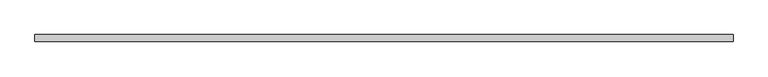
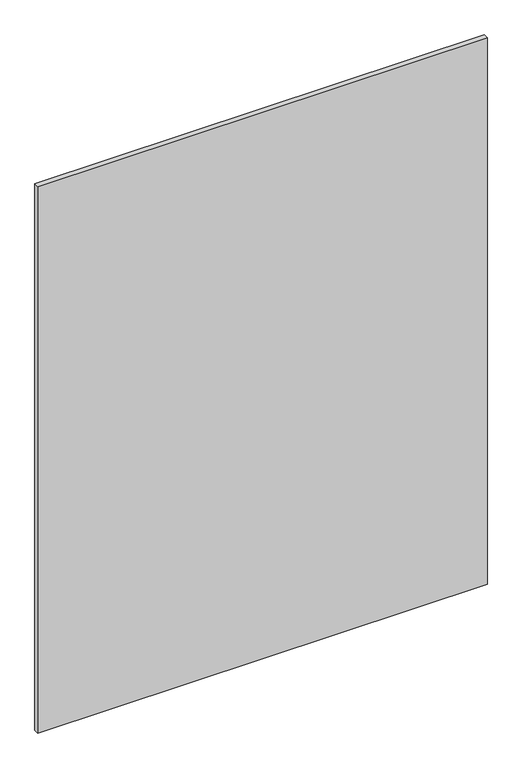
"""IFC4 building model written with IfcOpenShell, lengths in millimetres: proxy geometry, Vertical furring:Vertical furring:300288:Vertical furring:300288 : Vertical furring:Vertical furring:300288:300029:Vertical furring:300288:Vertical furring:300288 : Vertical furring:Vertical furring:300288:300029 : Vertical furring:Vertical furring:300288:Vertical furring:300288 : Vertical furring:Vertical furring:300288:300029:5 : Vertical furring:Vertical furring:300288:Vertical furring:300288 : Vertical furring:Vertical furring:300288:300029:Vertical furring:300288:Vertical furring:300288 : Vertical furring:Vertical furring:300288:300029 : Vertical furring:Vertical furring:300288:Vertical furring:300288 : Vertical furring:Vertical furring:300288:300029:300008."""

from ifc_helpers import new_model, si_unit, frame, origin, place, context, project, spatial, polyline, outline, extrude, source, transform, mapped, element, save


def generic_models_db998e1a(model_context):
    return source(origin(), model_context, "Body", "SweptSolid", [
        extrude(outline(polyline([(569170.5290705, -579019.7413841), (571062.2367239, -579019.7413841), (571062.2367239, -579038.7913841), (569170.5290705, -579038.7913841), (569170.5290705, -579019.7413841)])), frame((0.0, 0.0, 3731.7525972), z_axis=(0.0, 0.0, 1.0), x_axis=(1.0, 0.0, 0.0)), (0.0, 0.0, 1.0), 2429.279412),
    ])


if __name__ == "__main__":
    model = new_model("IFC4")
    model_context = context("Model", 3, world=origin())
    ifc_project = project(units=[si_unit("LENGTHUNIT", "METRE", prefix="MILLI")], contexts=[model_context])
    site = spatial("IfcSite", under=ifc_project)
    building = spatial("IfcBuilding", under=site)
    placement = place(None, origin())
    generic_models_shape = generic_models_db998e1a(model_context)
    element("IfcBuildingElementProxy", 1, Name="Vertical furring:Vertical furring:300288:Vertical furring:300288 : Vertical furring:Vertical furring:300288:300029:Vertical furring:300288:Vertical furring:300288 : Vertical furring:Vertical furring:300288:300029 : Vertical furring:Vertical furring:300288:Vertical furring:300288 : Vertical furring:Vertical furring:300288:300029:5 : Vertical furring:Vertical furring:300288:Vertical furring:300288 : Vertical furring:Vertical furring:300288:300029:Vertical furring:300288:Vertical furring:300288 : Vertical furring:Vertical furring:300288:300029 : Vertical furring:Vertical furring:300288:Vertical furring:300288 : Vertical furring:Vertical furring:300288:300029:300008", ObjectType="Vertical furring:Vertical furring:300288:Vertical furring:300288 : Vertical furring:Vertical furring:300288:300029:Vertical furring:300288:Vertical furring:300288 : Vertical furring:Vertical furring:300288:300029 : Vertical furring:Vertical furring:300288:Vertical furring:300288 : Vertical furring:Vertical furring:300288:300029:5 : Vertical furring:Vertical furring:300288:Vertical furring:300288 : Vertical furring:Vertical furring:300288:300029:Vertical furring:300288:Vertical furring:300288 : Vertical furring:Vertical furring:300288:300029 : Vertical furring:Vertical furring:300288:Vertical furring:300288 : Vertical furring:Vertical furring:300288:300029:300008", at=placement, inside=building, context=model_context, shape_type="MappedRepresentation", body=[
        mapped(generic_models_shape, transform((0.0, 0.0, 0.0), x_axis=(1.0, 0.0, 0.0), y_axis=(0.0, 1.0, 0.0), z_axis=(0.0, 0.0, 1.0))),
    ])
    save(model, "model.ifc")

# Revit data of these elements
# Type "Vertical furring:Vertical furring:300288:Vertical furring:300288 : Vertical furring:Vertical furring:300288:300029:Vertical furring:300288:Vertical furring:300288 : Vertical furring:Vertical furring:300288:300029 : Vertical furring:Vertical furring:300288:Vertical furring:300288 : Vertical furring:Vertical furring:300288:300029:5 : Vertical furring:Vertical furring:300288:Vertical furring:300288 : Vertical furring:Vertical furring:300288:300029:Vertical furring:300288:Vertical furring:300288 : Vertical furring:Vertical furring:300288:300029 : Vertical furring:Vertical furring:300288:Vertical furring:300288 : Vertical furring:Vertical furring:300288:300029:300008"
#   NameOverride = "Vertical furring:Vertical furring:300288:Vertical furring:300288 : Vertical furring:Vertical furring:300288:300029:Vertical furring:300288:Vertical furring:300288 : Vertical furring:Vertical furring:300288:300029 : Vertical furring:Vertical furring:300288:Vertical furring:300288 : Vertical furring:Vertical furring:300288:300029:300008"
#   ObjectTypeOverride = "Vertical furring:300288:Vertical furring:300288 : Vertical furring:Vertical furring:300288:300029 : Vertical furring:Vertical furring:300288:Vertical furring:300288 : Vertical furring:Vertical furring:300288:300029"
#   Reference = "Vertical furring"
#   Tag = "300008"
# Element 1 (IfcBuildingElementProxy, "Vertical furring:Vertical furring:300288:Vertical furring:300288 : Vertical furring:Vertical furring:300288:300029:Vertical furring:300288:Vertical furring:300288 : Vertical furring:Vertical furring:300288:300029 : Vertical furring:Vertical furring:300288:Vertical furring:300288 : Vertical furring:Vertical furring:300288:300029:5 : Vertical furring:Vertical furring:300288:Vertical furring:300288 : Vertical furring:Vertical furring:300288:300029:Vertical furring:300288:Vertical furring:300288 : Vertical furring:Vertical furring:300288:300029 : Vertical furring:Vertical furring:300288:Vertical furring:300288 : Vertical furring:Vertical furring:300288:300029:300008")
#   Materials on its faces: "1\" MINERAL WOOL BOARD INSULATION - BLACK MAT FACER"
# Materials
#   "1\" MINERAL WOOL BOARD INSULATION - BLACK MAT FACER": class "Unassigned", colour RGB 205 188 106, transparency 0, Cost = 0
